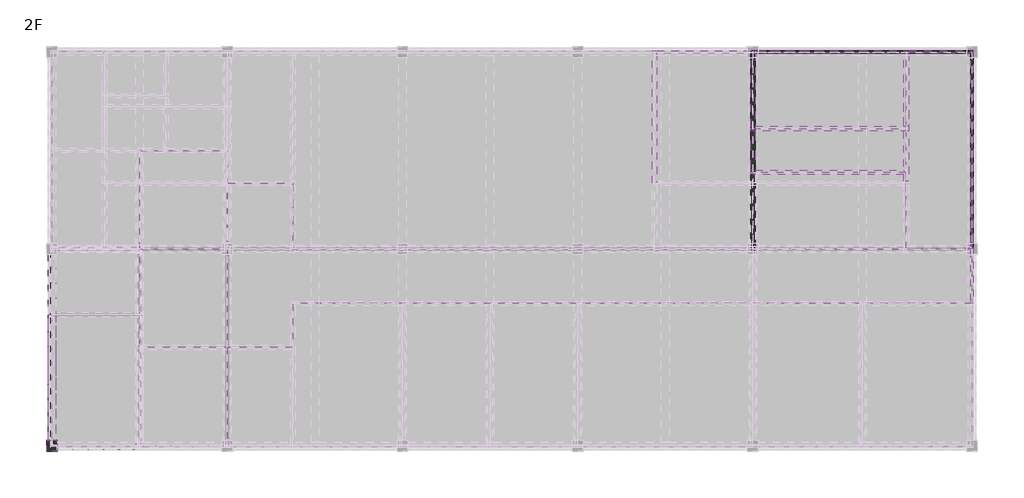
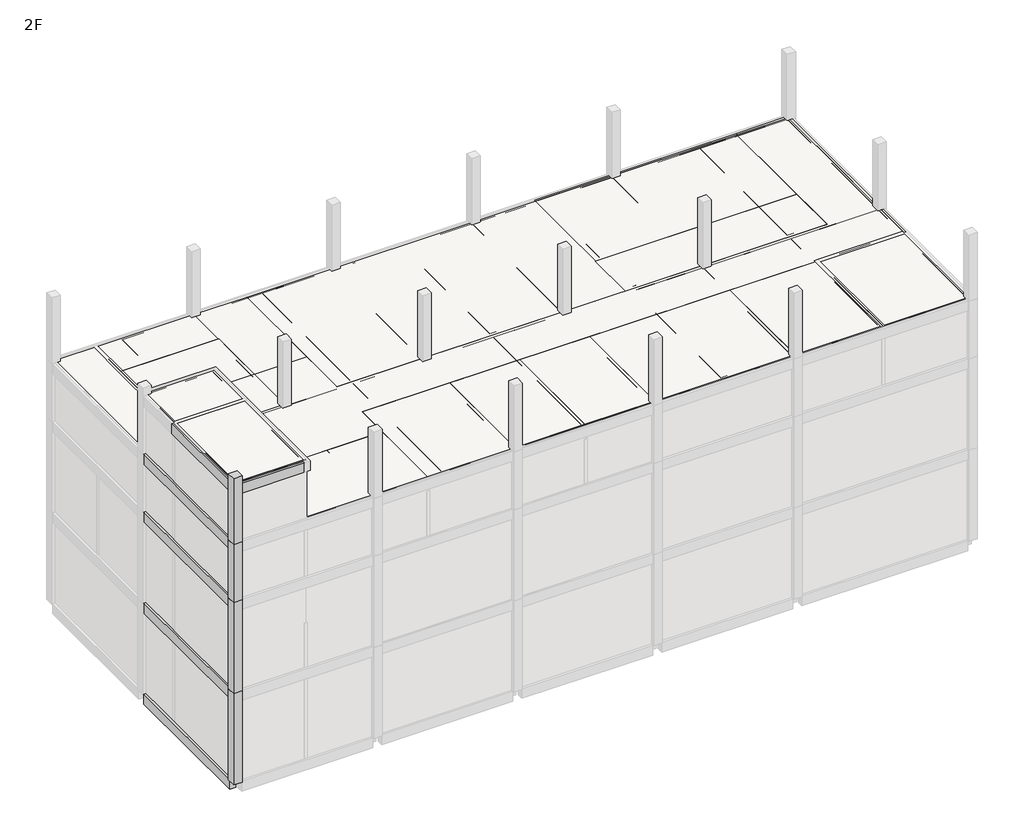
# One storey, part 3 of 7: 58 slabs, 16 walls, 6 beams, 4 columns.
"""IFC4 building model written with IfcOpenShell, lengths in millimetres."""

from ifc_helpers import new_model, si_unit, frame, origin, place, context, project, spatial, polyline, outline, extrude, faceted_brep, element, save

model = new_model("IFC4")

# Units and contexts
model_context = context("Model", 3, world=origin())
ifc_project = project(units=[si_unit("LENGTHUNIT", "METRE", prefix="MILLI")], contexts=[model_context])

# Site, building, storey
site = spatial("IfcSite", under=ifc_project)
building = spatial("IfcBuilding", under=site)
storey = spatial("IfcBuildingStorey", under=building, Name="2F", Elevation=3500.0)

# Beams
placement = place(None, origin())
element("IfcBeam", 1, ObjectType="Concrete-Rectangular-Beam : BM111_400x500_RG1", at=placement, inside=storey, context=model_context, shape_type="SweptSolid", body=[
    extrude(outline(polyline([(49284.6521483, 164098.8614395), (49284.6521483, 163748.8614395), (45709.6521483, 163748.8614395), (45709.6521483, 164098.8614395), (49284.6521483, 164098.8614395)])), frame((0.0, 0.0, 20900.0), z_axis=(0.0, 0.0, 1.0), x_axis=(1.0, 0.0, 0.0)), (0.0, 0.0, 1.0), 600.0),
])
element("IfcBeam", 2, ObjectType="Concrete-Rectangular-Beam : BM111_400x500_RG1", at=placement, inside=storey, context=model_context, shape_type="SweptSolid", body=[
    extrude(outline(polyline([(45284.6521483, 169923.8614395), (45634.6521483, 169923.8614395), (45634.6521483, 164173.8614395), (45284.6521483, 164173.8614395), (45284.6521483, 169923.8614395)])), frame((0.0, 0.0, 20900.0), z_axis=(0.0, 0.0, 1.0), x_axis=(1.0, 0.0, 0.0)), (0.0, 0.0, 1.0), 600.0),
])
element("IfcBeam", 3, ObjectType="Concrete-Rectangular-Beam : BM111_400x500_RG1", at=placement, inside=storey, context=model_context, shape_type="SweptSolid", body=[
    extrude(outline(polyline([(45284.6521483, 172673.8614395), (45634.6521483, 172673.8614395), (45634.6521483, 164173.8614395), (45284.6521483, 164173.8614395), (45284.6521483, 172673.8614395)])), frame((0.0, 0.0, 2900.0), z_axis=(0.0, 0.0, 1.0), x_axis=(1.0, 0.0, 0.0)), (0.0, 0.0, 1.0), 600.0),
])
element("IfcBeam", 4, ObjectType="Concrete-Rectangular-Beam : BM111_400x500_RG1", at=placement, inside=storey, context=model_context, shape_type="SweptSolid", body=[
    extrude(outline(polyline([(45284.6521483, 172673.8614395), (45634.6521483, 172673.8614395), (45634.6521483, 164173.8614395), (45284.6521483, 164173.8614395), (45284.6521483, 172673.8614395)])), frame((0.0, 0.0, 8400.0), z_axis=(0.0, 0.0, 1.0), x_axis=(1.0, 0.0, 0.0)), (0.0, 0.0, 1.0), 600.0),
])
element("IfcBeam", 5, ObjectType="Concrete-Rectangular-Beam : BM111_400x500_RG1", at=placement, inside=storey, context=model_context, shape_type="SweptSolid", body=[
    extrude(outline(polyline([(45284.6521483, 172673.8614395), (45634.6521483, 172673.8614395), (45634.6521483, 164173.8614395), (45284.6521483, 164173.8614395), (45284.6521483, 172673.8614395)])), frame((0.0, 0.0, 13900.0), z_axis=(0.0, 0.0, 1.0), x_axis=(1.0, 0.0, 0.0)), (0.0, 0.0, 1.0), 600.0),
])
element("IfcBeam", 6, ObjectType="Concrete-Rectangular-Beam : BM111_400x500_RG1", at=placement, inside=storey, context=model_context, shape_type="SweptSolid", body=[
    extrude(outline(polyline([(45284.6521483, 172673.8614395), (45634.6521483, 172673.8614395), (45634.6521483, 164173.8614395), (45284.6521483, 164173.8614395), (45284.6521483, 172673.8614395)])), frame((0.0, 0.0, 17400.0), z_axis=(0.0, 0.0, 1.0), x_axis=(1.0, 0.0, 0.0)), (0.0, 0.0, 1.0), 600.0),
])

# Columns
element("IfcColumn", 7, ObjectType="Concrete-Rectangular-Column : CL111_500x500", at=placement, inside=storey, context=model_context, shape_type="Brep", body=[
    faceted_brep([(45709.6521483, 164173.8614395, 3500.0), (45709.6521483, 163673.8614395, 3500.0), (45209.6521483, 163673.8614395, 3500.0), (45209.6521483, 164173.8614395, 3500.0), (45709.6521483, 164173.8614395, 9000.0), (45709.6521483, 164098.8614395, 9000.0), (45709.6521483, 163748.8614395, 9000.0), (45709.6521483, 163673.8614395, 9000.0), (45209.6521483, 163673.8614395, 9000.0), (45209.6521483, 164173.8614395, 9000.0), (45284.6521483, 164173.8614395, 9000.0), (45634.6521483, 164173.8614395, 9000.0)], [[[0, 1, 2, 3]], [[4, 5, 6, 7, 1, 0]], [[7, 8, 2, 1]], [[8, 9, 3, 2]], [[9, 10, 11, 4, 0, 3]], [[4, 11, 10, 9, 8, 7, 6, 5]]]),
])
element("IfcColumn", 8, ObjectType="Concrete-Rectangular-Column : CL111_500x500", at=placement, inside=storey, context=model_context, shape_type="Brep", body=[
    faceted_brep([(45709.6521483, 164173.8614395, 9000.0), (45709.6521483, 163673.8614395, 9000.0), (45209.6521483, 163673.8614395, 9000.0), (45209.6521483, 164173.8614395, 9000.0), (45709.6521483, 164173.8614395, 14500.0), (45709.6521483, 164098.8614395, 14500.0), (45709.6521483, 163748.8614395, 14500.0), (45709.6521483, 163673.8614395, 14500.0), (45209.6521483, 163673.8614395, 14500.0), (45209.6521483, 164173.8614395, 14500.0), (45284.6521483, 164173.8614395, 14500.0), (45634.6521483, 164173.8614395, 14500.0)], [[[0, 1, 2, 3]], [[4, 5, 6, 7, 1, 0]], [[7, 8, 2, 1]], [[8, 9, 3, 2]], [[9, 10, 11, 4, 0, 3]], [[4, 11, 10, 9, 8, 7, 6, 5]]]),
])
element("IfcColumn", 9, ObjectType="Concrete-Rectangular-Column : CL111_500x500", at=placement, inside=storey, context=model_context, shape_type="Brep", body=[
    faceted_brep([(45709.6521483, 164173.8614395, 14500.0), (45709.6521483, 163673.8614395, 14500.0), (45209.6521483, 163673.8614395, 14500.0), (45209.6521483, 164173.8614395, 14500.0), (45709.6521483, 164173.8614395, 18000.0), (45709.6521483, 164098.8614395, 18000.0), (45709.6521483, 163748.8614395, 18000.0), (45709.6521483, 163673.8614395, 18000.0), (45209.6521483, 163673.8614395, 18000.0), (45209.6521483, 164173.8614395, 18000.0), (45284.6521483, 164173.8614395, 18000.0), (45634.6521483, 164173.8614395, 18000.0)], [[[0, 1, 2, 3]], [[4, 5, 6, 7, 1, 0]], [[7, 8, 2, 1]], [[8, 9, 3, 2]], [[9, 10, 11, 4, 0, 3]], [[4, 11, 10, 9, 8, 7, 6, 5]]]),
])
element("IfcColumn", 10, ObjectType="Concrete-Rectangular-Column : CL111_500x500", at=placement, inside=storey, context=model_context, shape_type="SweptSolid", body=[
    extrude(outline(polyline([(45709.6521483, 164173.8614395), (45709.6521483, 163673.8614395), (45209.6521483, 163673.8614395), (45209.6521483, 164173.8614395), (45709.6521483, 164173.8614395)])), frame((0.0, 0.0, 18000.0), z_axis=(0.0, 0.0, 1.0), x_axis=(1.0, 0.0, 0.0)), (0.0, 0.0, 1.0), 4000.0),
])

# Slabs
element("IfcSlab", 11, ObjectType="CFS11_Slab RC_T150", at=placement, inside=storey, context=model_context, shape_type="SweptSolid", body=[
    extrude(outline(polyline([(77459.6521483, 181923.8614395), (77459.6521483, 172923.8614395), (45459.6521483, 172923.8614395), (45459.6521483, 181923.8614395), (77459.6521483, 181923.8614395)])), frame((0.0, 0.0, 3350.0), z_axis=(0.0, 0.0, 1.0), x_axis=(1.0, 0.0, 0.0)), (0.0, 0.0, 1.0), 150.0),
])
element("IfcSlab", 12, ObjectType="CFS11_Slab RC_T150", at=placement, inside=storey, context=model_context, shape_type="SweptSolid", body=[
    extrude(outline(polyline([(53459.6521483, 163923.8614395), (53459.6521483, 172923.8614395), (87459.6521483, 172923.8614395), (87459.6521483, 163923.8614395), (53459.6521483, 163923.8614395)])), frame((0.0, 0.0, 3350.0), z_axis=(0.0, 0.0, 1.0), x_axis=(1.0, 0.0, 0.0)), (0.0, 0.0, 1.0), 150.0),
])
element("IfcSlab", 13, ObjectType="CFS11_Slab RC_T150", at=placement, inside=storey, context=model_context, shape_type="SweptSolid", body=[
    extrude(outline(polyline([(77459.6521483, 181923.8614395), (87459.6521483, 181923.8614395), (87459.6521483, 172923.8614395), (77459.6521483, 172923.8614395), (77459.6521483, 181923.8614395)])), frame((0.0, 0.0, 3350.0), z_axis=(0.0, 0.0, 1.0), x_axis=(1.0, 0.0, 0.0)), (0.0, 0.0, 1.0), 150.0),
])
element("IfcSlab", 14, ObjectType="CFS11_Slab RC_T150", at=placement, inside=storey, context=model_context, shape_type="SweptSolid", body=[
    extrude(outline(polyline([(53459.6521483, 172923.8614395), (53459.6521483, 163923.8614395), (49459.6521483, 163923.8614395), (49459.6521483, 172923.8614395), (53459.6521483, 172923.8614395)])), frame((0.0, 0.0, 3350.0), z_axis=(0.0, 0.0, 1.0), x_axis=(1.0, 0.0, 0.0)), (0.0, 0.0, 1.0), 150.0),
])
element("IfcSlab", 15, ObjectType="CFS11_Slab RC_T150", at=placement, inside=storey, context=model_context, shape_type="SweptSolid", body=[
    extrude(outline(polyline([(49459.6521483, 172923.8614395), (49459.6521483, 169923.8614395), (45459.6521483, 169923.8614395), (45459.6521483, 172923.8614395), (49459.6521483, 172923.8614395)])), frame((0.0, 0.0, 3350.0), z_axis=(0.0, 0.0, 1.0), x_axis=(1.0, 0.0, 0.0)), (0.0, 0.0, 1.0), 150.0),
])
element("IfcSlab", 16, ObjectType="CFS11_Slab RC_T150", at=placement, inside=storey, context=model_context, shape_type="SweptSolid", body=[
    extrude(outline(polyline([(49459.6521483, 163923.8614395), (45459.6521483, 163923.8614395), (45459.6521483, 169923.8614395), (49459.6521483, 169923.8614395), (49459.6521483, 163923.8614395)])), frame((0.0, 0.0, 3350.0), z_axis=(0.0, 0.0, 1.0), x_axis=(1.0, 0.0, 0.0)), (0.0, 0.0, 1.0), 150.0),
])
element("IfcSlab", 17, ObjectType="CFS11_Slab RC_T150", at=placement, inside=storey, context=model_context, shape_type="SweptSolid", body=[
    extrude(outline(polyline([(53459.6521483, 181923.8614395), (77459.6521483, 181923.8614395), (77459.6521483, 172923.8614395), (53459.6521483, 172923.8614395), (53459.6521483, 181923.8614395)])), frame((0.0, 0.0, 8850.0), z_axis=(0.0, 0.0, 1.0), x_axis=(1.0, 0.0, 0.0)), (0.0, 0.0, 1.0), 150.0),
])
element("IfcSlab", 18, ObjectType="CFS11_Slab RC_T150", at=placement, inside=storey, context=model_context, shape_type="SweptSolid", body=[
    extrude(outline(polyline([(77459.6521483, 172923.8614395), (77459.6521483, 163923.8614395), (53459.6521483, 163923.8614395), (53459.6521483, 172923.8614395), (77459.6521483, 172923.8614395)])), frame((0.0, 0.0, 8850.0), z_axis=(0.0, 0.0, 1.0), x_axis=(1.0, 0.0, 0.0)), (0.0, 0.0, 1.0), 150.0),
])
element("IfcSlab", 19, ObjectType="CFS11_Slab RC_T150", at=placement, inside=storey, context=model_context, shape_type="SweptSolid", body=[
    extrude(outline(polyline([(77459.6521483, 181923.8614395), (84459.6521483, 181923.8614395), (84459.6521483, 178423.8614395), (77459.6521483, 178423.8614395), (77459.6521483, 181923.8614395)])), frame((0.0, 0.0, 8850.0), z_axis=(0.0, 0.0, 1.0), x_axis=(1.0, 0.0, 0.0)), (0.0, 0.0, 1.0), 150.0),
])
element("IfcSlab", 20, ObjectType="CFS11_Slab RC_T150", at=placement, inside=storey, context=model_context, shape_type="SweptSolid", body=[
    extrude(outline(polyline([(77459.6521483, 163923.8614395), (77459.6521483, 172923.8614395), (87459.6521483, 172923.8614395), (87459.6521483, 163923.8614395), (77459.6521483, 163923.8614395)])), frame((0.0, 0.0, 8850.0), z_axis=(0.0, 0.0, 1.0), x_axis=(1.0, 0.0, 0.0)), (0.0, 0.0, 1.0), 150.0),
])
element("IfcSlab", 21, ObjectType="CFS11_Slab RC_T150", at=placement, inside=storey, context=model_context, shape_type="SweptSolid", body=[
    extrude(outline(polyline([(77459.6521483, 176423.8614395), (84459.6521483, 176423.8614395), (84459.6521483, 172923.8614395), (77459.6521483, 172923.8614395), (77459.6521483, 176423.8614395)])), frame((0.0, 0.0, 8850.0), z_axis=(0.0, 0.0, 1.0), x_axis=(1.0, 0.0, 0.0)), (0.0, 0.0, 1.0), 150.0),
])
element("IfcSlab", 22, ObjectType="CFS11_Slab RC_T150", at=placement, inside=storey, context=model_context, shape_type="SweptSolid", body=[
    extrude(outline(polyline([(45459.6521483, 181923.8614395), (47859.6521483, 181923.8614395), (47859.6521483, 177423.8614395), (45459.6521483, 177423.8614395), (45459.6521483, 181923.8614395)])), frame((0.0, 0.0, 8850.0), z_axis=(0.0, 0.0, 1.0), x_axis=(1.0, 0.0, 0.0)), (0.0, 0.0, 1.0), 150.0),
])
element("IfcSlab", 23, ObjectType="CFS11_Slab RC_T150", at=placement, inside=storey, context=model_context, shape_type="SweptSolid", body=[
    extrude(outline(polyline([(45459.6521483, 172923.8614395), (45459.6521483, 177423.8614395), (49459.6521483, 177423.8614395), (49459.6521483, 172923.8614395), (45459.6521483, 172923.8614395)])), frame((0.0, 0.0, 8850.0), z_axis=(0.0, 0.0, 1.0), x_axis=(1.0, 0.0, 0.0)), (0.0, 0.0, 1.0), 150.0),
])
element("IfcSlab", 24, ObjectType="CFS11_Slab RC_T150", at=placement, inside=storey, context=model_context, shape_type="SweptSolid", body=[
    extrude(outline(polyline([(53459.6521483, 177423.8614395), (50659.6521483, 177423.8614395), (50659.6521483, 181923.8614395), (53459.6521483, 181923.8614395), (53459.6521483, 177423.8614395)])), frame((0.0, 0.0, 8850.0), z_axis=(0.0, 0.0, 1.0), x_axis=(1.0, 0.0, 0.0)), (0.0, 0.0, 1.0), 150.0),
])
element("IfcSlab", 25, ObjectType="CFS11_Slab RC_T150", at=placement, inside=storey, context=model_context, shape_type="SweptSolid", body=[
    extrude(outline(polyline([(47859.6521483, 181923.8614395), (50659.6521483, 181923.8614395), (50659.6521483, 179923.8614395), (47859.6521483, 179923.8614395), (47859.6521483, 181923.8614395)])), frame((0.0, 0.0, 8850.0), z_axis=(0.0, 0.0, 1.0), x_axis=(1.0, 0.0, 0.0)), (0.0, 0.0, 1.0), 150.0),
])
element("IfcSlab", 26, ObjectType="CFS11_Slab RC_T150", at=placement, inside=storey, context=model_context, shape_type="SweptSolid", body=[
    extrude(outline(polyline([(47859.6521483, 179923.8614395), (50659.6521483, 179923.8614395), (50659.6521483, 177423.8614395), (47859.6521483, 177423.8614395), (47859.6521483, 179923.8614395)])), frame((0.0, 0.0, 8850.0), z_axis=(0.0, 0.0, 1.0), x_axis=(1.0, 0.0, 0.0)), (0.0, 0.0, 1.0), 150.0),
])
element("IfcSlab", 27, ObjectType="CFS11_Slab RC_T150", at=placement, inside=storey, context=model_context, shape_type="SweptSolid", body=[
    extrude(outline(polyline([(49459.6521483, 172923.8614395), (49459.6521483, 169923.8614395), (45459.6521483, 169923.8614395), (45459.6521483, 172923.8614395), (49459.6521483, 172923.8614395)])), frame((0.0, 0.0, 8850.0), z_axis=(0.0, 0.0, 1.0), x_axis=(1.0, 0.0, 0.0)), (0.0, 0.0, 1.0), 150.0),
])
element("IfcSlab", 28, ObjectType="CFS11_Slab RC_T150", at=placement, inside=storey, context=model_context, shape_type="SweptSolid", body=[
    extrude(outline(polyline([(49459.6521483, 169923.8614395), (49459.6521483, 163923.8614395), (45459.6521483, 163923.8614395), (45459.6521483, 169923.8614395), (49459.6521483, 169923.8614395)])), frame((0.0, 0.0, 8850.0), z_axis=(0.0, 0.0, 1.0), x_axis=(1.0, 0.0, 0.0)), (0.0, 0.0, 1.0), 150.0),
])
element("IfcSlab", 29, ObjectType="CFS11_Slab RC_T150", at=placement, inside=storey, context=model_context, shape_type="SweptSolid", body=[
    extrude(outline(polyline([(77459.6521483, 178423.8614395), (84459.6521483, 178423.8614395), (84459.6521483, 181923.8614395), (87459.6521483, 181923.8614395), (87459.6521483, 172923.8614395), (84459.6521483, 172923.8614395), (84459.6521483, 176423.8614395), (77459.6521483, 176423.8614395), (77459.6521483, 178423.8614395)])), frame((0.0, 0.0, 8850.0), z_axis=(0.0, 0.0, 1.0), x_axis=(1.0, 0.0, 0.0)), (0.0, 0.0, 1.0), 150.0),
])
element("IfcSlab", 30, ObjectType="CFS11_Slab RC_T150", at=placement, inside=storey, context=model_context, shape_type="SweptSolid", body=[
    extrude(outline(polyline([(49459.6521483, 177423.8614395), (53459.6521483, 177423.8614395), (53459.6521483, 163923.8614395), (49459.6521483, 163923.8614395), (49459.6521483, 177423.8614395)])), frame((0.0, 0.0, 8850.0), z_axis=(0.0, 0.0, 1.0), x_axis=(1.0, 0.0, 0.0)), (0.0, 0.0, 1.0), 150.0),
])
element("IfcSlab", 31, ObjectType="CFS11_Slab RC_T150", at=placement, inside=storey, context=model_context, shape_type="SweptSolid", body=[
    extrude(outline(polyline([(61459.6521483, 163923.8614395), (61459.6521483, 170423.8614395), (65459.6521483, 170423.8614395), (65459.6521483, 163923.8614395), (61459.6521483, 163923.8614395)])), frame((0.0, 0.0, 14350.0), z_axis=(0.0, 0.0, 1.0), x_axis=(1.0, 0.0, 0.0)), (0.0, 0.0, 1.0), 150.0),
])
element("IfcSlab", 32, ObjectType="CFS11_Slab RC_T150", at=placement, inside=storey, context=model_context, shape_type="SweptSolid", body=[
    extrude(outline(polyline([(65459.6521483, 170423.8614395), (69459.6521483, 170423.8614395), (69459.6521483, 163923.8614395), (65459.6521483, 163923.8614395), (65459.6521483, 170423.8614395)])), frame((0.0, 0.0, 14350.0), z_axis=(0.0, 0.0, 1.0), x_axis=(1.0, 0.0, 0.0)), (0.0, 0.0, 1.0), 150.0),
])
element("IfcSlab", 33, ObjectType="CFS11_Slab RC_T150", at=placement, inside=storey, context=model_context, shape_type="SweptSolid", body=[
    extrude(outline(polyline([(84459.6521483, 181923.8614395), (84459.6521483, 175923.8614395), (72959.6521483, 175923.8614395), (72959.6521483, 181923.8614395), (84459.6521483, 181923.8614395)])), frame((0.0, 0.0, 14350.0), z_axis=(0.0, 0.0, 1.0), x_axis=(1.0, 0.0, 0.0)), (0.0, 0.0, 1.0), 150.0),
])
element("IfcSlab", 34, ObjectType="CFS11_Slab RC_T150", at=placement, inside=storey, context=model_context, shape_type="SweptSolid", body=[
    extrude(outline(polyline([(69459.6521483, 170423.8614395), (77459.6521483, 170423.8614395), (77459.6521483, 163923.8614395), (69459.6521483, 163923.8614395), (69459.6521483, 170423.8614395)])), frame((0.0, 0.0, 14350.0), z_axis=(0.0, 0.0, 1.0), x_axis=(1.0, 0.0, 0.0)), (0.0, 0.0, 1.0), 150.0),
])
element("IfcSlab", 35, ObjectType="CFS11_Slab RC_T150", at=placement, inside=storey, context=model_context, shape_type="SweptSolid", body=[
    extrude(outline(polyline([(56459.6521483, 181923.8614395), (72959.6521483, 181923.8614395), (72959.6521483, 172923.8614395), (56459.6521483, 172923.8614395), (56459.6521483, 181923.8614395)])), frame((0.0, 0.0, 14350.0), z_axis=(0.0, 0.0, 1.0), x_axis=(1.0, 0.0, 0.0)), (0.0, 0.0, 1.0), 150.0),
])
element("IfcSlab", 36, ObjectType="CFS11_Slab RC_T150", at=placement, inside=storey, context=model_context, shape_type="SweptSolid", body=[
    extrude(outline(polyline([(77459.6521483, 170423.8614395), (82459.6521483, 170423.8614395), (82459.6521483, 163923.8614395), (77459.6521483, 163923.8614395), (77459.6521483, 170423.8614395)])), frame((0.0, 0.0, 14350.0), z_axis=(0.0, 0.0, 1.0), x_axis=(1.0, 0.0, 0.0)), (0.0, 0.0, 1.0), 150.0),
])
element("IfcSlab", 37, ObjectType="CFS11_Slab RC_T150", at=placement, inside=storey, context=model_context, shape_type="SweptSolid", body=[
    extrude(outline(polyline([(82459.6521483, 170423.8614395), (87459.6521483, 170423.8614395), (87459.6521483, 163923.8614395), (82459.6521483, 163923.8614395), (82459.6521483, 170423.8614395)])), frame((0.0, 0.0, 14350.0), z_axis=(0.0, 0.0, 1.0), x_axis=(1.0, 0.0, 0.0)), (0.0, 0.0, 1.0), 150.0),
])
element("IfcSlab", 38, ObjectType="CFS11_Slab RC_T150", at=placement, inside=storey, context=model_context, shape_type="SweptSolid", body=[
    extrude(outline(polyline([(84459.6521483, 175923.8614395), (84459.6521483, 172923.8614395), (72959.6521483, 172923.8614395), (72959.6521483, 175923.8614395), (84459.6521483, 175923.8614395)])), frame((0.0, 0.0, 14350.0), z_axis=(0.0, 0.0, 1.0), x_axis=(1.0, 0.0, 0.0)), (0.0, 0.0, 1.0), 150.0),
])
element("IfcSlab", 39, ObjectType="CFS11_Slab RC_T150", at=placement, inside=storey, context=model_context, shape_type="SweptSolid", body=[
    extrude(outline(polyline([(61459.6521483, 163923.8614395), (56459.6521483, 163923.8614395), (56459.6521483, 170423.8614395), (61459.6521483, 170423.8614395), (61459.6521483, 163923.8614395)])), frame((0.0, 0.0, 14350.0), z_axis=(0.0, 0.0, 1.0), x_axis=(1.0, 0.0, 0.0)), (0.0, 0.0, 1.0), 150.0),
])
element("IfcSlab", 40, ObjectType="CFS11_Slab RC_T150", at=placement, inside=storey, context=model_context, shape_type="SweptSolid", body=[
    extrude(outline(polyline([(56459.6521483, 163923.8614395), (49459.6521483, 163923.8614395), (49459.6521483, 168423.8614395), (56459.6521483, 168423.8614395), (56459.6521483, 163923.8614395)])), frame((0.0, 0.0, 14350.0), z_axis=(0.0, 0.0, 1.0), x_axis=(1.0, 0.0, 0.0)), (0.0, 0.0, 1.0), 150.0),
])
element("IfcSlab", 41, ObjectType="CFS11_Slab RC_T150", at=placement, inside=storey, context=model_context, shape_type="SweptSolid", body=[
    extrude(outline(polyline([(53459.6521483, 179423.8614395), (53459.6521483, 175923.8614395), (47859.6521483, 175923.8614395), (47859.6521483, 179423.8614395), (53459.6521483, 179423.8614395)])), frame((0.0, 0.0, 14350.0), z_axis=(0.0, 0.0, 1.0), x_axis=(1.0, 0.0, 0.0)), (0.0, 0.0, 1.0), 150.0),
])
element("IfcSlab", 42, ObjectType="CFS11_Slab RC_T150", at=placement, inside=storey, context=model_context, shape_type="SweptSolid", body=[
    extrude(outline(polyline([(47859.6521483, 179423.8614395), (47859.6521483, 181923.8614395), (53459.6521483, 181923.8614395), (53459.6521483, 179423.8614395), (47859.6521483, 179423.8614395)])), frame((0.0, 0.0, 14350.0), z_axis=(0.0, 0.0, 1.0), x_axis=(1.0, 0.0, 0.0)), (0.0, 0.0, 1.0), 150.0),
])
element("IfcSlab", 43, ObjectType="CFS11_Slab RC_T150", at=placement, inside=storey, context=model_context, shape_type="SweptSolid", body=[
    extrude(outline(polyline([(56459.6521483, 175923.8614395), (53459.6521483, 175923.8614395), (53459.6521483, 181923.8614395), (56459.6521483, 181923.8614395), (56459.6521483, 175923.8614395)])), frame((0.0, 0.0, 14350.0), z_axis=(0.0, 0.0, 1.0), x_axis=(1.0, 0.0, 0.0)), (0.0, 0.0, 1.0), 150.0),
])
element("IfcSlab", 44, ObjectType="CFS11_Slab RC_T150", at=placement, inside=storey, context=model_context, shape_type="SweptSolid", body=[
    extrude(outline(polyline([(53459.6521483, 175923.8614395), (53459.6521483, 172923.8614395), (47859.6521483, 172923.8614395), (47859.6521483, 175923.8614395), (53459.6521483, 175923.8614395)])), frame((0.0, 0.0, 14350.0), z_axis=(0.0, 0.0, 1.0), x_axis=(1.0, 0.0, 0.0)), (0.0, 0.0, 1.0), 150.0),
])
element("IfcSlab", 45, ObjectType="CFS11_Slab RC_T150", at=placement, inside=storey, context=model_context, shape_type="SweptSolid", body=[
    extrude(outline(polyline([(45459.6521483, 181923.8614395), (47859.6521483, 181923.8614395), (47859.6521483, 172923.8614395), (45459.6521483, 172923.8614395), (45459.6521483, 181923.8614395)])), frame((0.0, 0.0, 14350.0), z_axis=(0.0, 0.0, 1.0), x_axis=(1.0, 0.0, 0.0)), (0.0, 0.0, 1.0), 150.0),
])
element("IfcSlab", 46, ObjectType="CFS11_Slab RC_T150", at=placement, inside=storey, context=model_context, shape_type="SweptSolid", body=[
    extrude(outline(polyline([(49459.6521483, 172923.8614395), (49459.6521483, 169923.8614395), (45459.6521483, 169923.8614395), (45459.6521483, 172923.8614395), (49459.6521483, 172923.8614395)])), frame((0.0, 0.0, 14350.0), z_axis=(0.0, 0.0, 1.0), x_axis=(1.0, 0.0, 0.0)), (0.0, 0.0, 1.0), 150.0),
])
element("IfcSlab", 47, ObjectType="CFS11_Slab RC_T150", at=placement, inside=storey, context=model_context, shape_type="SweptSolid", body=[
    extrude(outline(polyline([(49459.6521483, 163923.8614395), (45459.6521483, 163923.8614395), (45459.6521483, 169923.8614395), (49459.6521483, 169923.8614395), (49459.6521483, 163923.8614395)])), frame((0.0, 0.0, 14350.0), z_axis=(0.0, 0.0, 1.0), x_axis=(1.0, 0.0, 0.0)), (0.0, 0.0, 1.0), 150.0),
])
element("IfcSlab", 48, ObjectType="CFS11_Slab RC_T150", at=placement, inside=storey, context=model_context, shape_type="SweptSolid", body=[
    extrude(outline(polyline([(87459.6521483, 181923.8614395), (87459.6521483, 170423.8614395), (56459.6521483, 170423.8614395), (56459.6521483, 168423.8614395), (49459.6521483, 168423.8614395), (49459.6521483, 172923.8614395), (53459.6521483, 172923.8614395), (53459.6521483, 175923.8614395), (56459.6521483, 175923.8614395), (56459.6521483, 172923.8614395), (84459.6521483, 172923.8614395), (84459.6521483, 181923.8614395), (87459.6521483, 181923.8614395)])), frame((0.0, 0.0, 14350.0), z_axis=(0.0, 0.0, 1.0), x_axis=(1.0, 0.0, 0.0)), (0.0, 0.0, 1.0), 150.0),
])
element("IfcSlab", 49, ObjectType="CFS11_Slab RC_T150", at=placement, inside=storey, context=model_context, shape_type="SweptSolid", body=[
    extrude(outline(polyline([(45459.6521483, 172923.8614395), (49459.6521483, 172923.8614395), (49459.6521483, 169923.8614395), (45459.6521483, 169923.8614395), (45459.6521483, 172923.8614395)])), frame((0.0, 0.0, 17850.0), z_axis=(0.0, 0.0, 1.0), x_axis=(1.0, 0.0, 0.0)), (0.0, 0.0, 1.0), 150.0),
])
element("IfcSlab", 50, ObjectType="CFS11_Slab RC_T150", at=placement, inside=storey, context=model_context, shape_type="SweptSolid", body=[
    extrude(outline(polyline([(49459.6521483, 169923.8614395), (49459.6521483, 163923.8614395), (45459.6521483, 163923.8614395), (45459.6521483, 169923.8614395), (49459.6521483, 169923.8614395)])), frame((0.0, 0.0, 17850.0), z_axis=(0.0, 0.0, 1.0), x_axis=(1.0, 0.0, 0.0)), (0.0, 0.0, 1.0), 150.0),
])
element("IfcSlab", 51, ObjectType="CFS11_Slab RC_T150", at=placement, inside=storey, context=model_context, shape_type="SweptSolid", body=[
    extrude(outline(polyline([(61459.6521483, 163923.8614395), (61459.6521483, 170423.8614395), (65459.6521483, 170423.8614395), (65459.6521483, 163923.8614395), (61459.6521483, 163923.8614395)])), frame((0.0, 0.0, 17850.0), z_axis=(0.0, 0.0, 1.0), x_axis=(1.0, 0.0, 0.0)), (0.0, 0.0, 1.0), 150.0),
])
element("IfcSlab", 52, ObjectType="CFS11_Slab RC_T150", at=placement, inside=storey, context=model_context, shape_type="SweptSolid", body=[
    extrude(outline(polyline([(65459.6521483, 170423.8614395), (69459.6521483, 170423.8614395), (69459.6521483, 163923.8614395), (65459.6521483, 163923.8614395), (65459.6521483, 170423.8614395)])), frame((0.0, 0.0, 17850.0), z_axis=(0.0, 0.0, 1.0), x_axis=(1.0, 0.0, 0.0)), (0.0, 0.0, 1.0), 150.0),
])
element("IfcSlab", 53, ObjectType="CFS11_Slab RC_T150", at=placement, inside=storey, context=model_context, shape_type="SweptSolid", body=[
    extrude(outline(polyline([(84459.6521483, 181923.8614395), (84459.6521483, 175923.8614395), (72959.6521483, 175923.8614395), (72959.6521483, 181923.8614395), (84459.6521483, 181923.8614395)])), frame((0.0, 0.0, 17850.0), z_axis=(0.0, 0.0, 1.0), x_axis=(1.0, 0.0, 0.0)), (0.0, 0.0, 1.0), 150.0),
])
element("IfcSlab", 54, ObjectType="CFS11_Slab RC_T150", at=placement, inside=storey, context=model_context, shape_type="SweptSolid", body=[
    extrude(outline(polyline([(69459.6521483, 170423.8614395), (77459.6521483, 170423.8614395), (77459.6521483, 163923.8614395), (69459.6521483, 163923.8614395), (69459.6521483, 170423.8614395)])), frame((0.0, 0.0, 17850.0), z_axis=(0.0, 0.0, 1.0), x_axis=(1.0, 0.0, 0.0)), (0.0, 0.0, 1.0), 150.0),
])
element("IfcSlab", 55, ObjectType="CFS11_Slab RC_T150", at=placement, inside=storey, context=model_context, shape_type="SweptSolid", body=[
    extrude(outline(polyline([(56459.6521483, 181923.8614395), (72959.6521483, 181923.8614395), (72959.6521483, 172923.8614395), (56459.6521483, 172923.8614395), (56459.6521483, 181923.8614395)])), frame((0.0, 0.0, 17850.0), z_axis=(0.0, 0.0, 1.0), x_axis=(1.0, 0.0, 0.0)), (0.0, 0.0, 1.0), 150.0),
])
element("IfcSlab", 56, ObjectType="CFS11_Slab RC_T150", at=placement, inside=storey, context=model_context, shape_type="SweptSolid", body=[
    extrude(outline(polyline([(77459.6521483, 170423.8614395), (82459.6521483, 170423.8614395), (82459.6521483, 163923.8614395), (77459.6521483, 163923.8614395), (77459.6521483, 170423.8614395)])), frame((0.0, 0.0, 17850.0), z_axis=(0.0, 0.0, 1.0), x_axis=(1.0, 0.0, 0.0)), (0.0, 0.0, 1.0), 150.0),
])
element("IfcSlab", 57, ObjectType="CFS11_Slab RC_T150", at=placement, inside=storey, context=model_context, shape_type="SweptSolid", body=[
    extrude(outline(polyline([(82459.6521483, 170423.8614395), (87459.6521483, 170423.8614395), (87459.6521483, 163923.8614395), (82459.6521483, 163923.8614395), (82459.6521483, 170423.8614395)])), frame((0.0, 0.0, 17850.0), z_axis=(0.0, 0.0, 1.0), x_axis=(1.0, 0.0, 0.0)), (0.0, 0.0, 1.0), 150.0),
])
element("IfcSlab", 58, ObjectType="CFS11_Slab RC_T150", at=placement, inside=storey, context=model_context, shape_type="SweptSolid", body=[
    extrude(outline(polyline([(84459.6521483, 175923.8614395), (84459.6521483, 172923.8614395), (72959.6521483, 172923.8614395), (72959.6521483, 175923.8614395), (84459.6521483, 175923.8614395)])), frame((0.0, 0.0, 17850.0), z_axis=(0.0, 0.0, 1.0), x_axis=(1.0, 0.0, 0.0)), (0.0, 0.0, 1.0), 150.0),
])
element("IfcSlab", 59, ObjectType="CFS11_Slab RC_T150", at=placement, inside=storey, context=model_context, shape_type="SweptSolid", body=[
    extrude(outline(polyline([(61459.6521483, 163923.8614395), (56459.6521483, 163923.8614395), (56459.6521483, 170423.8614395), (61459.6521483, 170423.8614395), (61459.6521483, 163923.8614395)])), frame((0.0, 0.0, 17850.0), z_axis=(0.0, 0.0, 1.0), x_axis=(1.0, 0.0, 0.0)), (0.0, 0.0, 1.0), 150.0),
])
element("IfcSlab", 60, ObjectType="CFS11_Slab RC_T150", at=placement, inside=storey, context=model_context, shape_type="SweptSolid", body=[
    extrude(outline(polyline([(56459.6521483, 163923.8614395), (49459.6521483, 163923.8614395), (49459.6521483, 168423.8614395), (56459.6521483, 168423.8614395), (56459.6521483, 163923.8614395)])), frame((0.0, 0.0, 17850.0), z_axis=(0.0, 0.0, 1.0), x_axis=(1.0, 0.0, 0.0)), (0.0, 0.0, 1.0), 150.0),
])
element("IfcSlab", 61, ObjectType="CFS11_Slab RC_T150", at=placement, inside=storey, context=model_context, shape_type="SweptSolid", body=[
    extrude(outline(polyline([(53459.6521483, 179423.8614395), (53459.6521483, 175923.8614395), (47859.6521483, 175923.8614395), (47859.6521483, 179423.8614395), (53459.6521483, 179423.8614395)])), frame((0.0, 0.0, 17850.0), z_axis=(0.0, 0.0, 1.0), x_axis=(1.0, 0.0, 0.0)), (0.0, 0.0, 1.0), 150.0),
])
element("IfcSlab", 62, ObjectType="CFS11_Slab RC_T150", at=placement, inside=storey, context=model_context, shape_type="SweptSolid", body=[
    extrude(outline(polyline([(47859.6521483, 179423.8614395), (47859.6521483, 181923.8614395), (53459.6521483, 181923.8614395), (53459.6521483, 179423.8614395), (47859.6521483, 179423.8614395)])), frame((0.0, 0.0, 17850.0), z_axis=(0.0, 0.0, 1.0), x_axis=(1.0, 0.0, 0.0)), (0.0, 0.0, 1.0), 150.0),
])
element("IfcSlab", 63, ObjectType="CFS11_Slab RC_T150", at=placement, inside=storey, context=model_context, shape_type="SweptSolid", body=[
    extrude(outline(polyline([(56459.6521483, 175923.8614395), (53459.6521483, 175923.8614395), (53459.6521483, 181923.8614395), (56459.6521483, 181923.8614395), (56459.6521483, 175923.8614395)])), frame((0.0, 0.0, 17850.0), z_axis=(0.0, 0.0, 1.0), x_axis=(1.0, 0.0, 0.0)), (0.0, 0.0, 1.0), 150.0),
])
element("IfcSlab", 64, ObjectType="CFS11_Slab RC_T150", at=placement, inside=storey, context=model_context, shape_type="SweptSolid", body=[
    extrude(outline(polyline([(53459.6521483, 175923.8614395), (53459.6521483, 172923.8614395), (47859.6521483, 172923.8614395), (47859.6521483, 175923.8614395), (53459.6521483, 175923.8614395)])), frame((0.0, 0.0, 17850.0), z_axis=(0.0, 0.0, 1.0), x_axis=(1.0, 0.0, 0.0)), (0.0, 0.0, 1.0), 150.0),
])
element("IfcSlab", 65, ObjectType="CFS11_Slab RC_T150", at=placement, inside=storey, context=model_context, shape_type="SweptSolid", body=[
    extrude(outline(polyline([(45459.6521483, 181923.8614395), (47859.6521483, 181923.8614395), (47859.6521483, 172923.8614395), (45459.6521483, 172923.8614395), (45459.6521483, 181923.8614395)])), frame((0.0, 0.0, 17850.0), z_axis=(0.0, 0.0, 1.0), x_axis=(1.0, 0.0, 0.0)), (0.0, 0.0, 1.0), 150.0),
])
element("IfcSlab", 66, ObjectType="CFS11_Slab RC_T150", at=placement, inside=storey, context=model_context, shape_type="SweptSolid", body=[
    extrude(outline(polyline([(87459.6521483, 181923.8614395), (87459.6521483, 170423.8614395), (56459.6521483, 170423.8614395), (56459.6521483, 168423.8614395), (49459.6521483, 168423.8614395), (49459.6521483, 172923.8614395), (53459.6521483, 172923.8614395), (53459.6521483, 175923.8614395), (56459.6521483, 175923.8614395), (56459.6521483, 172923.8614395), (84459.6521483, 172923.8614395), (84459.6521483, 181923.8614395), (87459.6521483, 181923.8614395)])), frame((0.0, 0.0, 17850.0), z_axis=(0.0, 0.0, 1.0), x_axis=(1.0, 0.0, 0.0)), (0.0, 0.0, 1.0), 150.0),
])
element("IfcSlab", 67, ObjectType="CFS11_Slab RC_T150", at=placement, inside=storey, context=model_context, shape_type="SweptSolid", body=[
    extrude(outline(polyline([(45459.6521483, 172923.8614395), (49459.6521483, 172923.8614395), (49459.6521483, 169923.8614395), (45459.6521483, 169923.8614395), (45459.6521483, 172923.8614395)])), frame((0.0, 0.0, 21350.0), z_axis=(0.0, 0.0, 1.0), x_axis=(1.0, 0.0, 0.0)), (0.0, 0.0, 1.0), 150.0),
])
element("IfcSlab", 68, ObjectType="CFS11_Slab RC_T150", at=placement, inside=storey, context=model_context, shape_type="SweptSolid", body=[
    extrude(outline(polyline([(49459.6521483, 169923.8614395), (49459.6521483, 163923.8614395), (45459.6521483, 163923.8614395), (45459.6521483, 169923.8614395), (49459.6521483, 169923.8614395)])), frame((0.0, 0.0, 21350.0), z_axis=(0.0, 0.0, 1.0), x_axis=(1.0, 0.0, 0.0)), (0.0, 0.0, 1.0), 150.0),
])

# Walls
element("IfcWall", 69, ObjectType="WA211_Exterior-Cement Brick-90mm", at=placement, inside=storey, context=model_context, shape_type="Brep", body=[
    faceted_brep([(87402.6521483, 181980.8614395, 3500.0), (87402.6521483, 181866.8614395, 3500.0), (87402.6521483, 173030.8614395, 3500.0), (87402.6521483, 172923.8614395, 3500.0), (87402.6521483, 172923.8614395, 9000.0), (87402.6521483, 173030.8614395, 9000.0), (87402.6521483, 181866.8614395, 9000.0), (87402.6521483, 181980.8614395, 9000.0), (87516.6521483, 181980.8614395, 3500.0), (87516.6521483, 181980.8614395, 9000.0), (87516.6521483, 172923.8614395, 9000.0), (87516.6521483, 172923.8614395, 3500.0)], [[[0, 1, 2, 3, 4, 5, 6, 7]], [[8, 9, 10, 11]], [[3, 2, 1, 0, 8, 11]], [[4, 3, 11, 10]], [[7, 6, 5, 4, 10, 9]], [[0, 7, 9, 8]]]),
])
element("IfcWall", 70, ObjectType="WA211_Exterior-Cement Brick-90mm", at=placement, inside=storey, context=model_context, shape_type="SweptSolid", body=[
    extrude(outline(polyline([(87402.6521483, 181866.8614395), (77566.6521483, 181866.8614395), (77566.6521483, 181980.8614395), (87402.6521483, 181980.8614395), (87402.6521483, 181866.8614395)])), frame((0.0, 0.0, 3500.0), z_axis=(0.0, 0.0, 1.0), x_axis=(1.0, 0.0, 0.0)), (0.0, 0.0, 1.0), 5500.0),
])
element("IfcWall", 71, ObjectType="WA211_Exterior-Cement Brick-90mm", at=placement, inside=storey, context=model_context, shape_type="SweptSolid", body=[
    extrude(outline(polyline([(9000.0, 77566.6521483), (9000.0, 84352.6521483), (11700.0, 84352.6521483), (11700.0, 84459.6521483), (14500.0, 84459.6521483), (14500.0, 77459.6521483), (12400.0, 77459.6521483), (12400.0, 77566.6521483), (9000.0, 77566.6521483)])), frame((0.0, 181866.8614395, 0.0), z_axis=(0.0, 1.0, 0.0), x_axis=(0.0, 0.0, 1.0)), (0.0, 0.0, 1.0), 114.0),
])
element("IfcWall", 72, ObjectType="WA211_Exterior-Cement Brick-90mm", at=placement, inside=storey, context=model_context, shape_type="Brep", body=[
    faceted_brep([(87402.6521483, 181980.8614395, 9000.0), (87402.6521483, 181866.8614395, 9000.0), (87402.6521483, 173030.8614395, 9000.0), (87402.6521483, 172923.8614395, 9000.0), (87402.6521483, 172923.8614395, 14500.0), (87402.6521483, 173030.8614395, 14500.0), (87402.6521483, 181866.8614395, 14500.0), (87402.6521483, 181980.8614395, 14500.0), (87516.6521483, 181980.8614395, 9000.0), (87516.6521483, 181980.8614395, 14500.0), (87516.6521483, 172923.8614395, 14500.0), (87516.6521483, 172923.8614395, 9000.0)], [[[0, 1, 2, 3, 4, 5, 6, 7]], [[8, 9, 10, 11]], [[3, 2, 1, 0, 8, 11]], [[4, 3, 11, 10]], [[7, 6, 5, 4, 10, 9]], [[0, 7, 9, 8]]]),
])
element("IfcWall", 73, ObjectType="WA211_Exterior-Cement Brick-90mm", at=placement, inside=storey, context=model_context, shape_type="SweptSolid", body=[
    extrude(outline(polyline([(9000.0, 84566.6521483), (9000.0, 87402.6521483), (14500.0, 87402.6521483), (14500.0, 84459.6521483), (11700.0, 84459.6521483), (11700.0, 84566.6521483), (9000.0, 84566.6521483)])), frame((0.0, 181866.8614395, 0.0), z_axis=(0.0, 1.0, 0.0), x_axis=(0.0, 0.0, 1.0)), (0.0, 0.0, 1.0), 114.0),
])
element("IfcWall", 74, ObjectType="WA211_Exterior-Cement Brick-90mm", at=placement, inside=storey, context=model_context, shape_type="SweptSolid", body=[
    extrude(outline(polyline([(14500.0, 73066.6521483), (14500.0, 84352.6521483), (17200.0, 84352.6521483), (17200.0, 84459.6521483), (18000.0, 84459.6521483), (18000.0, 72959.6521483), (17200.0, 72959.6521483), (17200.0, 73066.6521483), (14500.0, 73066.6521483)])), frame((0.0, 181866.8614395, 0.0), z_axis=(0.0, 1.0, 0.0), x_axis=(0.0, 0.0, 1.0)), (0.0, 0.0, 1.0), 114.0),
])
element("IfcWall", 75, ObjectType="WA211_Exterior-Cement Brick-90mm", at=placement, inside=storey, context=model_context, shape_type="Brep", body=[
    faceted_brep([(87402.6521483, 181980.8614395, 14500.0), (87402.6521483, 181866.8614395, 14500.0), (87402.6521483, 170530.8614395, 14500.0), (87402.6521483, 170423.8614395, 14500.0), (87402.6521483, 170423.8614395, 18000.0), (87402.6521483, 170530.8614395, 18000.0), (87402.6521483, 181866.8614395, 18000.0), (87402.6521483, 181980.8614395, 18000.0), (87516.6521483, 181980.8614395, 14500.0), (87516.6521483, 181980.8614395, 18000.0), (87516.6521483, 170423.8614395, 18000.0), (87516.6521483, 170423.8614395, 14500.0)], [[[0, 1, 2, 3, 4, 5, 6, 7]], [[8, 9, 10, 11]], [[3, 2, 1, 0, 8, 11]], [[4, 3, 11, 10]], [[7, 6, 5, 4, 10, 9]], [[0, 7, 9, 8]]]),
])
element("IfcWall", 76, ObjectType="WA211_Exterior-Cement Brick-90mm", at=placement, inside=storey, context=model_context, shape_type="SweptSolid", body=[
    extrude(outline(polyline([(14500.0, 84566.6521483), (14500.0, 87402.6521483), (18000.0, 87402.6521483), (18000.0, 84459.6521483), (17200.0, 84459.6521483), (17200.0, 84566.6521483), (14500.0, 84566.6521483)])), frame((0.0, 181866.8614395, 0.0), z_axis=(0.0, 1.0, 0.0), x_axis=(0.0, 0.0, 1.0)), (0.0, 0.0, 1.0), 114.0),
])
element("IfcWall", 77, ObjectType="WA221_Interior-Cement Block-190mm", at=placement, inside=storey, context=model_context, shape_type="Brep", body=[
    faceted_brep([(77566.6521483, 172816.8614395, 3500.0), (77566.6521483, 173030.8614395, 3500.0), (77566.6521483, 181866.8614395, 3500.0), (77566.6521483, 181980.8614395, 3500.0), (77566.6521483, 181980.8614395, 9000.0), (77566.6521483, 181866.8614395, 9000.0), (77566.6521483, 173030.8614395, 9000.0), (77566.6521483, 172816.8614395, 9000.0), (77352.6521483, 172816.8614395, 3500.0), (77352.6521483, 172816.8614395, 9000.0), (77352.6521483, 173030.8614395, 9000.0), (77352.6521483, 181866.8614395, 9000.0), (77352.6521483, 181980.8614395, 9000.0), (77352.6521483, 181980.8614395, 3500.0), (77352.6521483, 181866.8614395, 3500.0), (77352.6521483, 173030.8614395, 3500.0)], [[[0, 1, 2, 3, 4, 5, 6, 7]], [[8, 9, 10, 11, 12, 13, 14, 15]], [[3, 2, 1, 0, 8, 15, 14, 13]], [[7, 6, 5, 4, 12, 11, 10, 9]], [[0, 7, 9, 8]], [[4, 3, 13, 12]]]),
])
element("IfcWall", 78, ObjectType="WA221_Interior-Cement Block-190mm", at=placement, inside=storey, context=model_context, shape_type="Brep", body=[
    faceted_brep([(77352.6521483, 181980.8614395, 9000.0), (77352.6521483, 181866.8614395, 9000.0), (77352.6521483, 178530.8614395, 9000.0), (77352.6521483, 178530.8614395, 11700.0), (77352.6521483, 178423.8614395, 11700.0), (77352.6521483, 178423.8614395, 12400.0), (77352.6521483, 181866.8614395, 12400.0), (77352.6521483, 181980.8614395, 12400.0), (77566.6521483, 181980.8614395, 9000.0), (77566.6521483, 181980.8614395, 12400.0), (77566.6521483, 181866.8614395, 12400.0), (77566.6521483, 178423.8614395, 12400.0), (77566.6521483, 178423.8614395, 11700.0), (77566.6521483, 178530.8614395, 11700.0), (77566.6521483, 178530.8614395, 9000.0), (77566.6521483, 181866.8614395, 9000.0), (77459.6521483, 181980.8614395, 12400.0)], [[[0, 1, 2, 3, 4, 5, 6, 7]], [[8, 9, 10, 11, 12, 13, 14, 15]], [[2, 1, 0, 8, 15, 14]], [[7, 6, 5, 11, 10, 9, 16]], [[0, 7, 16, 9, 8]], [[5, 4, 12, 11]], [[12, 4, 3, 13]], [[3, 2, 14, 13]]]),
])
element("IfcWall", 79, ObjectType="WA221_Interior-Cement Block-190mm", at=placement, inside=storey, context=model_context, shape_type="SweptSolid", body=[
    extrude(outline(polyline([(178316.8614395, 9000.0), (176530.8614395, 9000.0), (176530.8614395, 11700.0), (176423.8614395, 11700.0), (176423.8614395, 12400.0), (178423.8614395, 12400.0), (178423.8614395, 11700.0), (178316.8614395, 11700.0), (178316.8614395, 9000.0)])), frame((77352.6521483, 0.0, 0.0), z_axis=(1.0, 0.0, 0.0), x_axis=(0.0, 1.0, 0.0)), (0.0, 0.0, 1.0), 214.0),
])
element("IfcWall", 80, ObjectType="WA221_Interior-Cement Block-190mm", at=placement, inside=storey, context=model_context, shape_type="Brep", body=[
    faceted_brep([(84566.6521483, 178530.8614395, 9000.0), (84352.6521483, 178530.8614395, 9000.0), (77566.6521483, 178530.8614395, 9000.0), (77352.6521483, 178530.8614395, 9000.0), (77352.6521483, 178530.8614395, 11700.0), (77566.6521483, 178530.8614395, 11700.0), (84352.6521483, 178530.8614395, 11700.0), (84566.6521483, 178530.8614395, 11700.0), (84566.6521483, 178316.8614395, 9000.0), (84566.6521483, 178316.8614395, 11700.0), (77566.6521483, 178316.8614395, 11700.0), (77352.6521483, 178316.8614395, 11700.0), (77352.6521483, 178316.8614395, 9000.0), (77566.6521483, 178316.8614395, 9000.0), (77352.6521483, 178423.8614395, 11700.0)], [[[0, 1, 2, 3, 4, 5, 6, 7]], [[8, 9, 10, 11, 12, 13]], [[3, 2, 1, 0, 8, 13, 12]], [[7, 6, 5, 4, 14, 11, 10, 9]], [[0, 7, 9, 8]], [[4, 3, 12, 11, 14]]]),
])
element("IfcWall", 81, ObjectType="WA221_Interior-Cement Block-190mm", at=placement, inside=storey, context=model_context, shape_type="Brep", body=[
    faceted_brep([(84352.6521483, 181980.8614395, 9000.0), (84352.6521483, 181866.8614395, 9000.0), (84352.6521483, 178530.8614395, 9000.0), (84352.6521483, 178530.8614395, 11700.0), (84352.6521483, 181866.8614395, 11700.0), (84352.6521483, 181980.8614395, 11700.0), (84566.6521483, 181980.8614395, 9000.0), (84566.6521483, 181980.8614395, 11700.0), (84566.6521483, 181866.8614395, 11700.0), (84566.6521483, 178530.8614395, 11700.0), (84566.6521483, 178530.8614395, 9000.0), (84566.6521483, 181866.8614395, 9000.0), (84459.6521483, 181980.8614395, 11700.0)], [[[0, 1, 2, 3, 4, 5]], [[6, 7, 8, 9, 10, 11]], [[2, 1, 0, 6, 11, 10]], [[5, 4, 3, 9, 8, 7, 12]], [[0, 5, 12, 7, 6]], [[3, 2, 10, 9]]]),
])
element("IfcWall", 82, ObjectType="WA221_Interior-Cement Block-190mm", at=placement, inside=storey, context=model_context, shape_type="Brep", body=[
    faceted_brep([(84352.6521483, 176530.8614395, 9000.0), (77566.6521483, 176530.8614395, 9000.0), (77352.6521483, 176530.8614395, 9000.0), (77352.6521483, 176530.8614395, 11700.0), (77566.6521483, 176530.8614395, 11700.0), (84352.6521483, 176530.8614395, 11700.0), (84352.6521483, 176316.8614395, 9000.0), (84352.6521483, 176316.8614395, 11700.0), (77566.6521483, 176316.8614395, 11700.0), (77352.6521483, 176316.8614395, 11700.0), (77352.6521483, 176316.8614395, 9000.0), (77566.6521483, 176316.8614395, 9000.0), (77352.6521483, 176423.8614395, 11700.0)], [[[0, 1, 2, 3, 4, 5]], [[6, 7, 8, 9, 10, 11]], [[2, 1, 0, 6, 11, 10]], [[5, 4, 3, 12, 9, 8, 7]], [[3, 2, 10, 9, 12]], [[0, 5, 7, 6]]]),
])
element("IfcWall", 83, ObjectType="WA221_Interior-Cement Block-190mm", at=placement, inside=storey, context=model_context, shape_type="Brep", body=[
    faceted_brep([(73066.6521483, 175923.8614395, 14500.0), (73066.6521483, 176030.8614395, 14500.0), (73066.6521483, 181866.8614395, 14500.0), (73066.6521483, 181980.8614395, 14500.0), (73066.6521483, 181980.8614395, 17200.0), (73066.6521483, 181866.8614395, 17200.0), (73066.6521483, 176030.8614395, 17200.0), (73066.6521483, 175923.8614395, 17200.0), (72852.6521483, 175923.8614395, 14500.0), (72852.6521483, 175923.8614395, 17200.0), (72852.6521483, 181866.8614395, 17200.0), (72852.6521483, 181980.8614395, 17200.0), (72852.6521483, 181980.8614395, 14500.0), (72852.6521483, 181866.8614395, 14500.0), (72959.6521483, 181980.8614395, 17200.0)], [[[0, 1, 2, 3, 4, 5, 6, 7]], [[8, 9, 10, 11, 12, 13]], [[3, 2, 1, 0, 8, 13, 12]], [[7, 6, 5, 4, 14, 11, 10, 9]], [[0, 7, 9, 8]], [[4, 3, 12, 11, 14]]]),
])
element("IfcWall", 84, ObjectType="WA221_Interior-Cement Block-190mm", at=placement, inside=storey, context=model_context, shape_type="Brep", body=[
    faceted_brep([(84352.6521483, 181980.8614395, 14500.0), (84352.6521483, 181866.8614395, 14500.0), (84352.6521483, 176030.8614395, 14500.0), (84352.6521483, 176030.8614395, 17200.0), (84352.6521483, 181866.8614395, 17200.0), (84352.6521483, 181980.8614395, 17200.0), (84566.6521483, 181980.8614395, 14500.0), (84566.6521483, 181980.8614395, 17200.0), (84566.6521483, 181866.8614395, 17200.0), (84566.6521483, 176030.8614395, 17200.0), (84566.6521483, 176030.8614395, 14500.0), (84566.6521483, 181866.8614395, 14500.0), (84459.6521483, 181980.8614395, 17200.0)], [[[0, 1, 2, 3, 4, 5]], [[6, 7, 8, 9, 10, 11]], [[2, 1, 0, 6, 11, 10]], [[5, 4, 3, 9, 8, 7, 12]], [[0, 5, 12, 7, 6]], [[3, 2, 10, 9]]]),
])

save(model, "model.ifc")

# Revit data of these elements
# Type "Concrete-Rectangular-Beam : BM111_400x500_RG1"
#   중앙부 하부근 = "3-D20"
#   중앙부 상부근 = "3-D20"
#   중앙부 보조근 = ""
#   중앙부 늑근 = "2-D10 @200"
#   외단부 하부근 = "3-D20"
#   외단부 상부근 = "3-D20"
#   외단부 보조근 = ""
#   외단부 늑근 = "2-D10 @100"
#   부호 = "RG1"
#   내단부 하부근 = "3-D20"
#   내단부 상부근 = "3-D20"
#   내단부 보조근 = ""
#   내단부 늑근 = "2-D10 @100"
#   ALL 하부근 = ""
#   ALL 상부근 = ""
#   ALL 보조근 = ""
#   ALL 늑근 = ""
#   Width = 400 mm
#   Height = 500 mm
#   Length [instance default] = 1524 mm
#   Structural Material [instance default] = 콘크리트 - 현장타설 콘크리트
#   hec_material3 [instance default] = none
#   hec_material2 [instance default] = none
#   hec_material1 [instance default] = none
#   Assembly Code = ""
# Type "Concrete-Rectangular-Column : CL111_500x500"
#   Description = "UG 철골 기둥용 Pedestal"
#   b = 500 mm
#   h = 500 mm
#   hec_material3 [instance default] = none
#   hec_material2 [instance default] = A03AE056-00001_Bitumen/Bituminous/Asphalt Coating
#   hec_material1 [instance default] = A03AC035-00001_Form Work (3 times in use)_Flat
#   Structural Material [instance default] = A03AC032-00007_Structural Concrete_Type1_25MPa-30Mpa
# Type "CFS11_Slab RC_T150"
#   Keynote = ""
#   Type Comments = "구조_콘크리트"
#   Function = 0
#   Layers, outside or top first: 150 mm "14200-030101_Concrete Pouring" (function 1)
# Type "WA211_Exterior-Cement Brick-90mm"
#   Type Comments = ""
#   Layers, outside or top first: 0 mm "A04AL081-00001_Skirt_Acrylic Emulsion Paint" (function 100); 0 mm "A04AL077-00001_Ext Wall Painting_Acrylic Emulsion Paint" (function 100); 12 mm "A04AS164-00001_Plastering_Ext" (function 4); 90 mm "A04AK073-00001_Concrete Brick_0.5B" (function 1); 12 mm "A04AS164-00002_Plastering_Int" (function 5); 0 mm "A04AL078-00002_Int Wall Painting_Water Emulsion Paint" (function 100); 0 mm "A04AL081-00001_Skirt_Acrylic Emulsion Paint" (function 100)
# Type "WA221_Interior-Cement Block-190mm"
#   Type Comments = ""
#   Layers, outside or top first: 0 mm "A04AL081-00001_Skirt_Acrylic Emulsion Paint" (function 100); 0 mm "A04AL078-00002_Int Wall Painting_Water Emulsion Paint" (function 100); 12 mm "A04AS164-00002_Plastering_Int" (function 2); 190 mm "A04AK069-00002_Reinforced Concrete Block_THK 100-200mm" (function 1); 12 mm "A04AS164-00002_Plastering_Int" (function 2); 0 mm "A04AL078-00002_Int Wall Painting_Water Emulsion Paint" (function 100); 0 mm "A04AL081-00001_Skirt_Acrylic Emulsion Paint" (function 100)
# Elements 1, 2, 3, 4, 5, 6 (IfcBeam, "Concrete-Rectangular-Beam : BM111_400x500_RG1")
#   Comments = ""
#   hec_material3 = none
#   hec_material2 = none
#   hec_material1 = none
#   Structural Material = 콘크리트 - 현장타설 콘크리트
#   Phase Created = New Construction
#   Materials on its faces: "콘크리트 - 현장타설 콘크리트"
# Elements 7, 8, 9, 10 (IfcColumn, "Concrete-Rectangular-Column : CL111_500x500")
#   Comments = ""
#   hec_material3 = none
#   hec_material2 = none
#   hec_material1 = none
#   Structural Material = 콘크리트 - 현장타설 콘크리트
#   Phase Created = New Construction
#   Materials on its faces: "콘크리트 - 현장타설 콘크리트"
# Elements 11, 12, 13, 14, 15, 16, 17, 18, 19, 20, 21, 22, 23, 24, 25, 26, 27, 28, 29, 30, 31, 32, 33, 34, 35, 36, 37, 38, 39, 40, 41, 42, 43, 44, 45, 46, 47, 48, 49, 50 (IfcSlab, "CFS11_Slab RC_T150")
#   Height Offset From Level = 0 mm
#   Phase Created = New Construction
#   Materials on its faces: "14200-030101_Concrete Pouring"
# Elements 51, 52, 53, 54, 55, 56, 57, 58, 59, 60, 61, 62, 63, 64, 65, 66, 67, 68 (IfcSlab, "CFS11_Slab RC_T150")
#   Height Offset From Level = 3500 mm
#   Phase Created = New Construction
#   Materials on its faces: "14200-030101_Concrete Pouring"
# Element 69 (IfcWall, "WA211_Exterior-Cement Brick-90mm")
#   Top Offset = 0 mm
#   Base Offset = 0 mm
#   Unconnected Height = 5500 mm
#   wall height = 5500 mm
#   Phase Created = New Construction
#   Base Constraint = 2F
#   Materials on its faces: "Default Wall", "A04AS164-00001_Plastering_Ext", "A04AS164-00002_Plastering_Int"
# Element 70 (IfcWall, "WA211_Exterior-Cement Brick-90mm")
#   Top Offset = 0 mm
#   Base Offset = 0 mm
#   Unconnected Height = 5500 mm
#   wall height = 5500 mm
#   Phase Created = New Construction
#   Base Constraint = 2F
#   Materials on its faces: "Default Wall", "A04AS164-00002_Plastering_Int", "A04AS164-00001_Plastering_Ext"
# Elements 71, 73 (IfcWall, "WA211_Exterior-Cement Brick-90mm")
#   Top Offset = 0 mm
#   Base Offset = 0 mm
#   Unconnected Height = 5500 mm
#   wall height = 5500 mm
#   Phase Created = New Construction
#   Base Constraint = 3F
#   Materials on its faces: "Default Wall", "A04AS164-00002_Plastering_Int", "A04AS164-00001_Plastering_Ext"
# Element 72 (IfcWall, "WA211_Exterior-Cement Brick-90mm")
#   Top Offset = 0 mm
#   Base Offset = 0 mm
#   Unconnected Height = 5500 mm
#   wall height = 5500 mm
#   Phase Created = New Construction
#   Base Constraint = 3F
#   Materials on its faces: "Default Wall", "A04AS164-00001_Plastering_Ext", "A04AS164-00002_Plastering_Int"
# Elements 74, 76 (IfcWall, "WA211_Exterior-Cement Brick-90mm")
#   Top Offset = 0 mm
#   Base Offset = 0 mm
#   Unconnected Height = 3500 mm
#   wall height = 3500 mm
#   Phase Created = New Construction
#   Base Constraint = 4F
#   Materials on its faces: "Default Wall", "A04AS164-00002_Plastering_Int", "A04AS164-00001_Plastering_Ext"
# Element 75 (IfcWall, "WA211_Exterior-Cement Brick-90mm")
#   Top Offset = 0 mm
#   Base Offset = 0 mm
#   Unconnected Height = 3500 mm
#   wall height = 3500 mm
#   Phase Created = New Construction
#   Base Constraint = 4F
#   Materials on its faces: "Default Wall", "A04AS164-00001_Plastering_Ext", "A04AS164-00002_Plastering_Int"
# Element 77 (IfcWall, "WA221_Interior-Cement Block-190mm")
#   Top Offset = 0 mm
#   Base Offset = 0 mm
#   Unconnected Height = 5500 mm
#   wall height = 5500 mm
#   Phase Created = New Construction
#   Base Constraint = 2F
#   Materials on its faces: "A04AS164-00002_Plastering_Int", "Default Wall", "A04AS164-00001_Plastering_Ext"
# Element 78 (IfcWall, "WA221_Interior-Cement Block-190mm")
#   Top Offset = 0 mm
#   Base Offset = 0 mm
#   Unconnected Height = 3400 mm
#   wall height = 3400 mm
#   Phase Created = New Construction
#   Base Constraint = 3F
#   Materials on its faces: "Default Wall", "A04AS164-00002_Plastering_Int", "A04AS164-00001_Plastering_Ext"
# Element 79 (IfcWall, "WA221_Interior-Cement Block-190mm")
#   Top Offset = 0 mm
#   Base Offset = 0 mm
#   Unconnected Height = 3400 mm
#   wall height = 3400 mm
#   Phase Created = New Construction
#   Base Constraint = 3F
#   Materials on its faces: "Default Wall", "A04AS164-00002_Plastering_Int"
# Elements 80, 82 (IfcWall, "WA221_Interior-Cement Block-190mm")
#   Top Offset = 0 mm
#   Base Offset = 0 mm
#   Unconnected Height = 2700 mm
#   wall height = 2700 mm
#   Phase Created = New Construction
#   Base Constraint = 3F
#   Materials on its faces: "A04AS164-00002_Plastering_Int", "Default Wall"
# Element 81 (IfcWall, "WA221_Interior-Cement Block-190mm")
#   Top Offset = 0 mm
#   Base Offset = 0 mm
#   Unconnected Height = 2700 mm
#   wall height = 2700 mm
#   Phase Created = New Construction
#   Base Constraint = 3F
#   Materials on its faces: "Default Wall", "A04AS164-00002_Plastering_Int", "A04AS164-00001_Plastering_Ext"
# Elements 83, 84 (IfcWall, "WA221_Interior-Cement Block-190mm")
#   Top Offset = 0 mm
#   Base Offset = 0 mm
#   Unconnected Height = 2700 mm
#   wall height = 2700 mm
#   Phase Created = New Construction
#   Base Constraint = 4F
#   Materials on its faces: "Default Wall", "A04AS164-00002_Plastering_Int", "A04AS164-00001_Plastering_Ext"
# Materials
#   "콘크리트 - 현장타설 콘크리트": class "콘크리트", colour RGB 192 192 192, transparency 0
#   "A03AE056-00001_Bitumen/Bituminous/Asphalt Coating": class "Generic", colour RGB 17 17 17, transparency 0, Description = "Damp-proofing", W00) Work Master Code = "A03AE056-00001", W01) Work Master_Lv1 = "Concrete Work", W02) Work Master_Lv2 = "Concrete Protective Coating (U/G)", W03) Work Master_Spec.1 = "Bitumen/Bituminous/Asphalt Coating", Cost = 0
#   "A03AC035-00001_Form Work (3 times in use)_Flat": class "Wood", colour RGB 149 120 74, transparency 0, Description = "Plywood", W00) Work Master Code = "A03AC035-00001", W01) Work Master_Lv1 = "Concrete Work", W02) Work Master_Lv2 = "Substructure Work", W03) Work Master_Spec.1 = "Form Work (3 times in use)", W04) Work Master_Spec.2 = "Flat Form", W05) Work Master_Spec.3 = "Dressed Lumber, Plywood or Steel Form(Wood Planks are not Allowed) incl. Chamfer", Cost = 0
#   "A03AC032-00007_Structural Concrete_Type1_25MPa-30Mpa": class "Concrete", colour RGB 176 176 176, transparency 0, Keynote = "09910.A1", Description = "Reinf. Conc.", W00) Work Master Code = "A03AC032-00007", W01) Work Master_Lv1 = "Concrete Work", W02) Work Master_Lv2 = "Substructure Work", W03) Work Master_Spec.1 = "Structural Concrete", W04) Work Master_Spec.2 = "Cement Type-1", W05) Work Master_Spec.3 = "25MPa < F'c (Cylinder Strength) ≤ 30MPa", Cost = 0
#   "14200-030101_Concrete Pouring": class "Concrete", colour RGB 176 176 176, transparency 0, Description = "Reinf. Conc.", W00) Work Master Code = "14200-030101", W01) Work Master_Lv1 = "Concrete Work", W02) Work Master_Lv2 = "Building/Shelter Foundation Work", W03) Work Master_Spec.1 = "Concrete Pouring", W04) Work Master_Spec.2 = "F'c (Cylinder Strength) > 35MPa", W05) Work Master_Spec.3 = "Cement Type-1", Cost = 0
#   "A04AL081-00001_Skirt_Acrylic Emulsion Paint": class "Finish", colour RGB 128 128 64, transparency 0, Description = "Plastic", W00) Work Master Code = "A04AL081-00001", W01) Work Master_Lv1 = "Finishing Work", W02) Work Master_Lv2 = "Painting Work", W03) Work Master_Spec.1 = "Skirt Painting", W04) Work Master_Spec.2 = "Acrylic Emulsion Paint", W05) Work Master_Spec.3 = "100mm≤H<150mm", Cost = 0
#   "A04AL077-00001_Ext Wall Painting_Acrylic Emulsion Paint": class "Finish", colour RGB 128 128 64, transparency 0, Description = "Plastic", W00) Work Master Code = "A04AL077-00001", W01) Work Master_Lv1 = "Finishing Work", W02) Work Master_Lv2 = "Painting Work", W03) Work Master_Spec.1 = "External Wall Painting", W04) Work Master_Spec.2 = "Acrylic Emulsion Paint", Cost = 0
